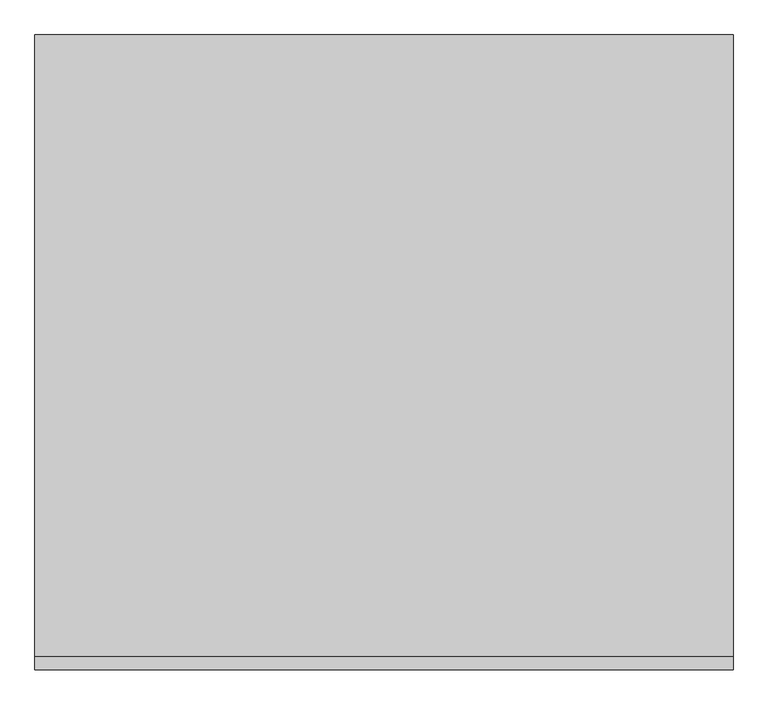
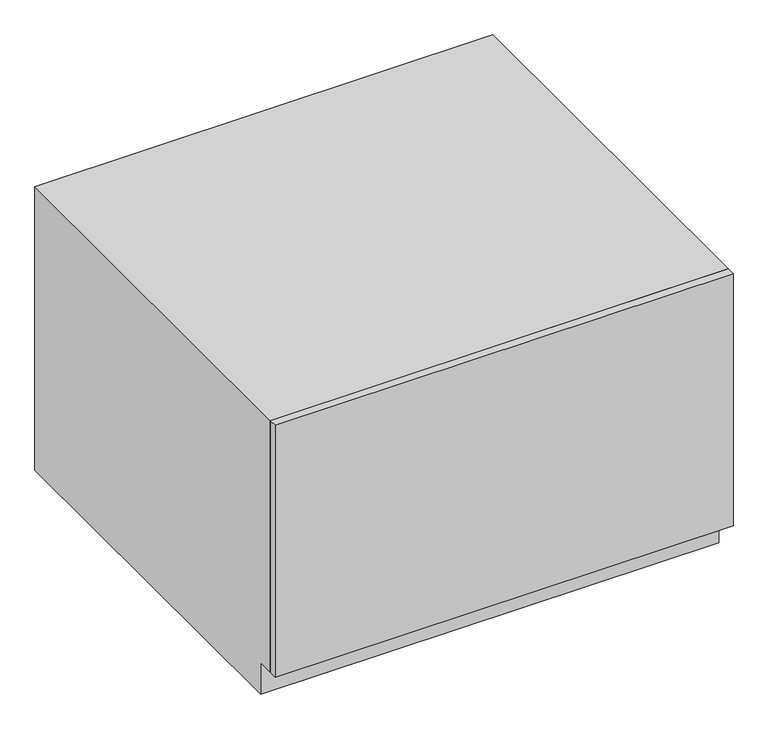
"""IFC4 building model written with IfcOpenShell, lengths in millimetres: furniture geometry, OD_CW_Base Cabinet : OD_CW_Base Cabinet."""

import ifcopenshell
import ifcopenshell.guid

model = None  # the IFC model being written
_history = None  # IfcOwnerHistory: only IFC2X3 demands one
_inside = {}  # id of a spatial element -> (the spatial element, [elements in it])
_under = {}  # id of a project, library or spatial element -> (it, [spatial elements below it])
_declared = {}  # id of a project -> (the project, [libraries it declares])
_typed = {}  # id of a type object -> (the type object, [elements of that type])
_made_of = {}  # id of a material, layer set ... -> (it, [elements and type objects made of it])


def new_model(schema):
    """Start an empty IFC model of exactly this schema.

    Asked for "IFC4X3", IfcOpenShell would pick the latest addendum, in which some entities
    have other attributes; the version numbers below select the first issue.
    IFC2X3 requires an IfcOwnerHistory on every rooted entity: one is made here for all.
    """
    global model, _history
    if schema == "IFC4X3":
        model = ifcopenshell.file(schema_version=(4, 3, 0, 0))
    else:
        model = ifcopenshell.file(schema=schema)
    _inside.clear()
    _under.clear()
    _declared.clear()
    _typed.clear()
    _made_of.clear()
    _history = None
    if model.schema == "IFC2X3":
        org = make("IfcOrganization", Name="unknown")
        user = make(
            "IfcPersonAndOrganization",
            ThePerson=make("IfcPerson", FamilyName="unknown"),
            TheOrganization=org,
        )
        app = make(
            "IfcApplication",
            ApplicationDeveloper=org,
            Version="unknown",
            ApplicationFullName="unknown",
            ApplicationIdentifier="unknown",
        )
        _history = make(
            "IfcOwnerHistory",
            OwningUser=user,
            OwningApplication=app,
            ChangeAction="ADDED",
            CreationDate=0,
        )
    return model


def make(cls, **values):
    """One entity of the class cls with the attributes given. An attribute that is None is left unset."""
    return model.create_entity(
        cls, **{name: value for name, value in values.items() if value is not None}
    )


def rooted(cls, **values):
    """An entity with a GlobalId (a new one), such as an element, a storey or a relation."""
    return make(cls, GlobalId=ifcopenshell.guid.new(), OwnerHistory=_history, **values)


def si_unit(unit_type, name, prefix=None):
    """IfcSIUnit, for example si_unit("LENGTHUNIT", "METRE", prefix="MILLI")."""
    return make("IfcSIUnit", UnitType=unit_type, Prefix=prefix, Name=name)


def assignment(units):
    """IfcUnitAssignment: the units of a project."""
    return None if units is None else make("IfcUnitAssignment", Units=units)


def point(xyz):
    """IfcCartesianPoint."""
    return None if xyz is None else make("IfcCartesianPoint", Coordinates=xyz)


def direction(xyz):
    """IfcDirection."""
    return None if xyz is None else make("IfcDirection", DirectionRatios=xyz)


def frame(location, z_axis=None, x_axis=None):
    """IfcAxis2Placement3D, a coordinate frame: its origin and axes. An axis left out is left unset."""
    return make(
        "IfcAxis2Placement3D",
        Location=point(location),
        Axis=direction(z_axis),
        RefDirection=direction(x_axis),
    )


def origin():
    """The frame at (0, 0, 0) with its axes left unset."""
    return frame((0.0, 0.0, 0.0))


def place(relative_to, where):
    """IfcLocalPlacement: puts the frame where relative to a parent placement (None: the world)."""
    return make(
        "IfcLocalPlacement", PlacementRelTo=relative_to, RelativePlacement=where
    )


def context(
    kind, dimensions, precision=None, world=None, true_north=None, identifier=None
):
    """IfcGeometricRepresentationContext, for example the 3D "Model" context."""
    return make(
        "IfcGeometricRepresentationContext",
        ContextIdentifier=identifier,
        ContextType=kind,
        CoordinateSpaceDimension=dimensions,
        Precision=precision,
        WorldCoordinateSystem=world,
        TrueNorth=true_north,
    )


def project(units=None, contexts=None):
    """IfcProject with its units and contexts."""
    return rooted(
        "IfcProject",
        Name="project",
        RepresentationContexts=contexts,
        UnitsInContext=assignment(units),
    )


def spatial(cls, under=None, at=None, **own):
    """A site, building, storey or space (cls), placed at a placement, below another one or the project."""
    s = rooted(cls, ObjectPlacement=at, **own)
    if under is not None:
        _under.setdefault(under.id(), (under, []))[1].append(s)
    return s


def polyline(points):
    """IfcPolyline through the points."""
    return make("IfcPolyline", Points=[point(p) for p in points])


def outline(outer, holes=None, kind="AREA"):
    """IfcArbitraryClosedProfileDef: a profile drawn as a closed curve; with holes, ...WithVoids."""
    if holes is None:
        return make("IfcArbitraryClosedProfileDef", ProfileType=kind, OuterCurve=outer)
    return make(
        "IfcArbitraryProfileDefWithVoids",
        ProfileType=kind,
        OuterCurve=outer,
        InnerCurves=holes,
    )


def extrude(swept, where, along, depth):
    """IfcExtrudedAreaSolid: the profile swept, set in the frame where, extruded along a direction by depth."""
    return make(
        "IfcExtrudedAreaSolid",
        SweptArea=swept,
        Position=where,
        ExtrudedDirection=direction(along),
        Depth=depth,
    )


def shape(context_of_items, identifier, shape_type, items):
    """IfcShapeRepresentation: the items that make up one representation, for example the "Body"."""
    return make(
        "IfcShapeRepresentation",
        ContextOfItems=context_of_items,
        RepresentationIdentifier=identifier,
        RepresentationType=shape_type,
        Items=items,
    )


def source(mapping_origin, context_of_items, identifier, shape_type, items):
    """IfcRepresentationMap: a shape defined once, which mapped items show again and again."""
    return make(
        "IfcRepresentationMap",
        MappingOrigin=mapping_origin,
        MappedRepresentation=shape(context_of_items, identifier, shape_type, items),
    )


def transform(
    local_origin,
    x_axis=None,
    y_axis=None,
    z_axis=None,
    scale=None,
    scale2=None,
    scale3=None,
    uniform=True,
):
    """IfcCartesianTransformationOperator3D, or its non-uniform kind. x_axis, y_axis, z_axis: its Axis1, 2, 3."""
    if uniform:
        return make(
            "IfcCartesianTransformationOperator3D",
            Axis1=direction(x_axis),
            Axis2=direction(y_axis),
            LocalOrigin=point(local_origin),
            Scale=scale,
            Axis3=direction(z_axis),
        )
    return make(
        "IfcCartesianTransformationOperator3DnonUniform",
        Axis1=direction(x_axis),
        Axis2=direction(y_axis),
        LocalOrigin=point(local_origin),
        Scale=scale,
        Axis3=direction(z_axis),
        Scale2=scale2,
        Scale3=scale3,
    )


def mapped(mapping_source, mapping_target):
    """IfcMappedItem: shows the shape of a source again, moved by a transform."""
    return make(
        "IfcMappedItem", MappingSource=mapping_source, MappingTarget=mapping_target
    )


def made_of(thing, what):
    """Note that an element or type object is made of a material, layer set ...; save() writes the relation."""
    if what is not None:
        _made_of.setdefault(what.id(), (what, []))[1].append(thing)
    return thing


def element(
    cls,
    number,
    at=None,
    inside=None,
    cuts=None,
    type_object=None,
    material=None,
    context=None,
    identifier="Body",
    shape_type=None,
    held_by="IfcProductDefinitionShape",
    body=None,
    shapes=None,
    **own,
):
    """One element of the class cls, such as IfcWall. Its Tag is "e" and its number.

    at: its placement. inside: the storey or other place that contains it. cuts: it is an
    opening in that element (IfcRelVoidsElement). A single representation is given by context,
    identifier, shape_type and body (its items); several are given by shapes. held_by: the class
    of the entity that holds the representations. save() writes the other relations.
    """
    e = rooted(cls, Tag="e%d" % number, ObjectPlacement=at, **own)
    if body is not None:
        shapes = [shape(context, identifier, shape_type, body)]
    if shapes is not None:
        e.Representation = make(held_by, Representations=shapes)
    if inside is not None:
        _inside.setdefault(inside.id(), (inside, []))[1].append(e)
    if cuts is not None:
        rooted(
            "IfcRelVoidsElement", RelatingBuildingElement=cuts, RelatedOpeningElement=e
        )
    if type_object is not None:
        _typed.setdefault(type_object.id(), (type_object, []))[1].append(e)
    return made_of(e, material)


def aggregate(whole, parts):
    """IfcRelAggregates: a whole, such as a stair, and the parts it consists of."""
    return rooted("IfcRelAggregates", RelatingObject=whole, RelatedObjects=parts)


def save(model, path):
    """Write the relations noted so far, then the file.

    IfcRelAggregates (storeys below a building ...), IfcRelContainedInSpatialStructure (elements
    in a storey), IfcRelDefinesByType, IfcRelAssociatesMaterial and IfcRelDeclares: one each for
    every whole, place, type object, material and project.
    """
    for whole, parts in _under.values():
        aggregate(whole, parts)
    for where, things in _inside.values():
        rooted(
            "IfcRelContainedInSpatialStructure",
            RelatedElements=things,
            RelatingStructure=where,
        )
    for kind, things in _typed.values():
        rooted("IfcRelDefinesByType", RelatedObjects=things, RelatingType=kind)
    for what, things in _made_of.values():
        rooted("IfcRelAssociatesMaterial", RelatedObjects=things, RelatingMaterial=what)
    for by, libraries in _declared.values():
        rooted("IfcRelDeclares", RelatingContext=by, RelatedDefinitions=libraries)
    model.write(path)


def furniture_86b526d0(model_context):
    return source(origin(), model_context, "Body", "SweptSolid", [
        extrude(outline(polyline([(18.7377049, -635.0), (1415.7377049, -635.0), (1415.7377049, -660.4), (18.7377049, -660.4), (18.7377049, -635.0)])), frame((0.0, 0.0, 101.6), z_axis=(0.0, 0.0, 1.0), x_axis=(1.0, 0.0, 0.0)), (0.0, 0.0, 1.0), 812.8),
        extrude(outline(polyline([(-635.0, 914.4), (609.6, 914.4), (609.6, 0.0), (-584.2, 0.0), (-584.2, 101.6), (-635.0, 101.6), (-635.0, 914.4)])), frame((18.7377049, 0.0, 0.0), z_axis=(1.0, 0.0, 0.0), x_axis=(0.0, 1.0, 0.0)), (0.0, 0.0, 1.0), 1397.0),
    ])


if __name__ == "__main__":
    model = new_model("IFC4")
    model_context = context("Model", 3, world=origin())
    ifc_project = project(units=[si_unit("LENGTHUNIT", "METRE", prefix="MILLI")], contexts=[model_context])
    site = spatial("IfcSite", under=ifc_project)
    building = spatial("IfcBuilding", under=site)
    placement = place(None, origin())
    furniture_shape = furniture_86b526d0(model_context)
    element("IfcFurniture", 1, ObjectType="OD_CW_Base Cabinet : OD_CW_Base Cabinet", at=placement, inside=building, context=model_context, shape_type="MappedRepresentation", body=[
        mapped(furniture_shape, transform((0.0, 0.0, 0.0), x_axis=(1.0, 0.0, 0.0), y_axis=(0.0, 1.0, 0.0), z_axis=(0.0, 0.0, 1.0))),
    ])
    save(model, "model.ifc")

# Revit data of these elements
# Type "OD_CW_Base Cabinet : OD_CW_Base Cabinet"
#   OD_CW_Width [instance default] = 2' - 10"
#   OD_CW_Length [instance default] = 8' - 0"
#   OD_CW_Height [instance default] = 2' - 3"
#   Depth = 2' - 0"
#   Height = 3' - 0"
#   Width = 4' - 0"
#   OD_CW_Material_Front Panel [instance default] = none
#   OD_CW_Material_Body [instance default] = none
# Element 1 (IfcFurniture, "OD_CW_Base Cabinet : OD_CW_Base Cabinet")
#   OD_CW_Width = 4' - 2"
#   OD_CW_Length = 4' - 7"
#   OD_CW_Height = 3' - 0"
#   OD_CW_Material_Body = CUPPONE PIZZA OVEN
#   Materials on its faces: "CUPPONE PIZZA OVEN", "CASEWORK"
# Materials
#   "CUPPONE PIZZA OVEN": class "Generic", colour RGB 187 187 187, transparency 0, Cost = 0
#   "CASEWORK": class "Generic", colour RGB 181 181 181, transparency 0, Cost = 0
